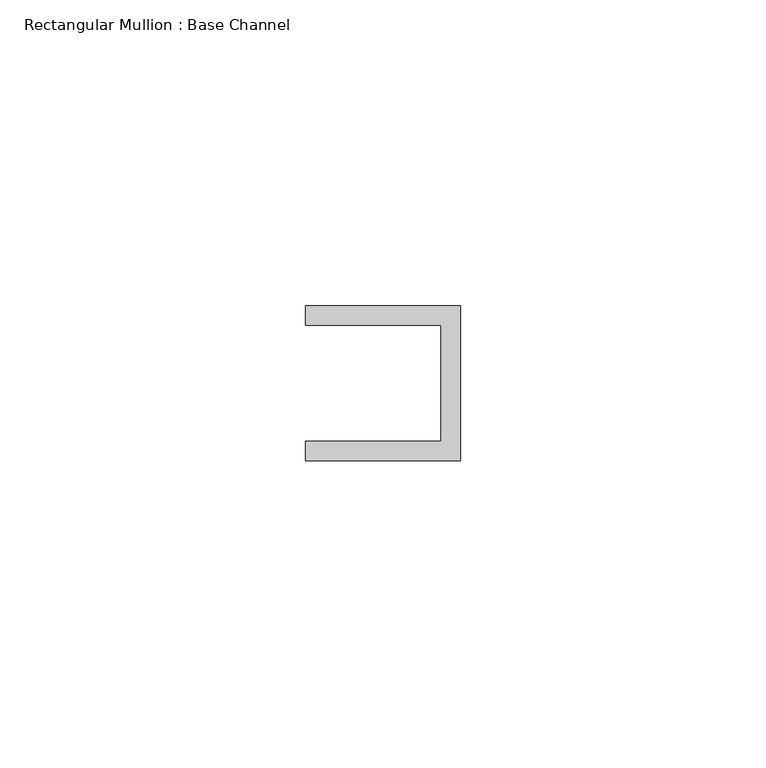
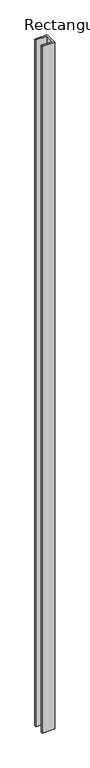
"""IFC4 building model written with IfcOpenShell, lengths in millimetres: member geometry, Rectangular Mullion : Base Channel."""

from ifc_helpers import new_model, si_unit, frame, origin, place, context, project, spatial, polyline, outline, extrude, source, transform, mapped, element, save


def rectangular_mullion_base_channel_b35d6865(model_context):
    return source(origin(), model_context, "Body", "SweptSolid", [
        extrude(outline(polyline([(0.0, -12.7), (-25.4, -12.7), (-25.4, -9.525), (-3.175, -9.525), (-3.175, 9.525), (-25.4, 9.525), (-25.4, 12.7), (0.0, 12.7), (0.0, -12.7)])), frame((0.0, 0.0, -1466.8372391), z_axis=(0.0, 0.0, 1.0), x_axis=(1.0, 0.0, 0.0)), (0.0, 0.0, 1.0), 1466.8372391),
    ])


if __name__ == "__main__":
    model = new_model("IFC4")
    model_context = context("Model", 3, world=origin())
    ifc_project = project(units=[si_unit("LENGTHUNIT", "METRE", prefix="MILLI")], contexts=[model_context])
    site = spatial("IfcSite", under=ifc_project)
    building = spatial("IfcBuilding", under=site)
    placement = place(None, origin())
    rectangular_mullion_base_channel_shape = rectangular_mullion_base_channel_b35d6865(model_context)
    element("IfcMember", 1, ObjectType="Rectangular Mullion : Base Channel", at=placement, inside=building, context=model_context, shape_type="MappedRepresentation", body=[
        mapped(rectangular_mullion_base_channel_shape, transform((0.0, 0.0, 0.0), x_axis=(1.0, 0.0, 0.0), y_axis=(0.0, 1.0, 0.0), z_axis=(0.0, 0.0, 1.0))),
    ])
    save(model, "model.ifc")

# Revit data of these elements
# Type "Rectangular Mullion : Base Channel"
#   built-in parameter 1007322 = 0.0833333 (stored number, unit not read)
#   built-in parameter 1007321 = 0.0416667 (stored number, unit not read)
#   built-in parameter 1007320 = -0.03125 (stored number, unit not read)
# Element 1 (IfcMember, "Rectangular Mullion : Base Channel")
#   Materials on its faces: "ALUM"
# Materials
#   "ALUM": class "Generic", colour RGB 157 157 157, transparency 0, Cost = 0
